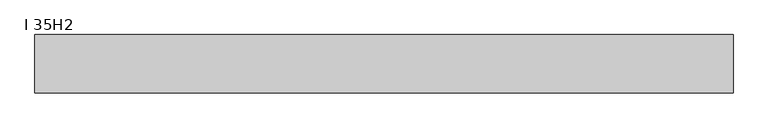
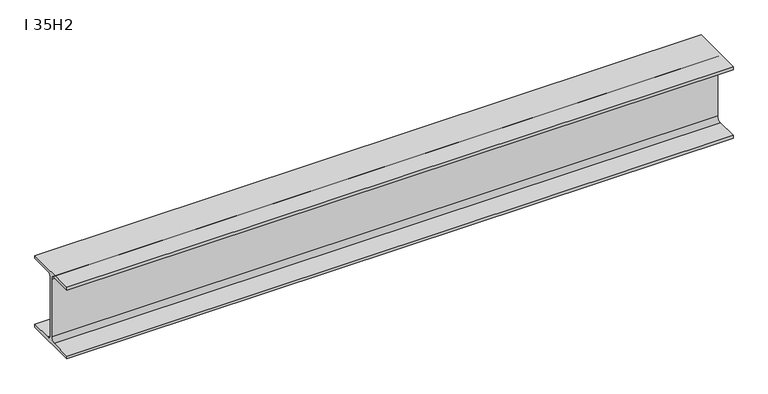
"""IFC4 building model written with IfcOpenShell, lengths in millimetres: beam geometry, Двутавр широкополочный (ГОСТ 26020-83) : I 35H2."""

import ifcopenshell
import ifcopenshell.guid

model = None  # the IFC model being written
_history = None  # IfcOwnerHistory: only IFC2X3 demands one
_inside = {}  # id of a spatial element -> (the spatial element, [elements in it])
_under = {}  # id of a project, library or spatial element -> (it, [spatial elements below it])
_declared = {}  # id of a project -> (the project, [libraries it declares])
_typed = {}  # id of a type object -> (the type object, [elements of that type])
_made_of = {}  # id of a material, layer set ... -> (it, [elements and type objects made of it])


def new_model(schema):
    """Start an empty IFC model of exactly this schema.

    Asked for "IFC4X3", IfcOpenShell would pick the latest addendum, in which some entities
    have other attributes; the version numbers below select the first issue.
    IFC2X3 requires an IfcOwnerHistory on every rooted entity: one is made here for all.
    """
    global model, _history
    if schema == "IFC4X3":
        model = ifcopenshell.file(schema_version=(4, 3, 0, 0))
    else:
        model = ifcopenshell.file(schema=schema)
    _inside.clear()
    _under.clear()
    _declared.clear()
    _typed.clear()
    _made_of.clear()
    _history = None
    if model.schema == "IFC2X3":
        org = make("IfcOrganization", Name="unknown")
        user = make(
            "IfcPersonAndOrganization",
            ThePerson=make("IfcPerson", FamilyName="unknown"),
            TheOrganization=org,
        )
        app = make(
            "IfcApplication",
            ApplicationDeveloper=org,
            Version="unknown",
            ApplicationFullName="unknown",
            ApplicationIdentifier="unknown",
        )
        _history = make(
            "IfcOwnerHistory",
            OwningUser=user,
            OwningApplication=app,
            ChangeAction="ADDED",
            CreationDate=0,
        )
    return model


def make(cls, **values):
    """One entity of the class cls with the attributes given. An attribute that is None is left unset."""
    return model.create_entity(
        cls, **{name: value for name, value in values.items() if value is not None}
    )


def rooted(cls, **values):
    """An entity with a GlobalId (a new one), such as an element, a storey or a relation."""
    return make(cls, GlobalId=ifcopenshell.guid.new(), OwnerHistory=_history, **values)


def si_unit(unit_type, name, prefix=None):
    """IfcSIUnit, for example si_unit("LENGTHUNIT", "METRE", prefix="MILLI")."""
    return make("IfcSIUnit", UnitType=unit_type, Prefix=prefix, Name=name)


def assignment(units):
    """IfcUnitAssignment: the units of a project."""
    return None if units is None else make("IfcUnitAssignment", Units=units)


def point(xyz):
    """IfcCartesianPoint."""
    return None if xyz is None else make("IfcCartesianPoint", Coordinates=xyz)


def direction(xyz):
    """IfcDirection."""
    return None if xyz is None else make("IfcDirection", DirectionRatios=xyz)


def frame(location, z_axis=None, x_axis=None):
    """IfcAxis2Placement3D, a coordinate frame: its origin and axes. An axis left out is left unset."""
    return make(
        "IfcAxis2Placement3D",
        Location=point(location),
        Axis=direction(z_axis),
        RefDirection=direction(x_axis),
    )


def frame_2d(location, x_axis=None):
    """IfcAxis2Placement2D, a coordinate frame in the plane: its origin and x axis."""
    return make(
        "IfcAxis2Placement2D", Location=point(location), RefDirection=direction(x_axis)
    )


def origin():
    """The frame at (0, 0, 0) with its axes left unset."""
    return frame((0.0, 0.0, 0.0))


def place(relative_to, where):
    """IfcLocalPlacement: puts the frame where relative to a parent placement (None: the world)."""
    return make(
        "IfcLocalPlacement", PlacementRelTo=relative_to, RelativePlacement=where
    )


def context(
    kind, dimensions, precision=None, world=None, true_north=None, identifier=None
):
    """IfcGeometricRepresentationContext, for example the 3D "Model" context."""
    return make(
        "IfcGeometricRepresentationContext",
        ContextIdentifier=identifier,
        ContextType=kind,
        CoordinateSpaceDimension=dimensions,
        Precision=precision,
        WorldCoordinateSystem=world,
        TrueNorth=true_north,
    )


def project(units=None, contexts=None):
    """IfcProject with its units and contexts."""
    return rooted(
        "IfcProject",
        Name="project",
        RepresentationContexts=contexts,
        UnitsInContext=assignment(units),
    )


def spatial(cls, under=None, at=None, **own):
    """A site, building, storey or space (cls), placed at a placement, below another one or the project."""
    s = rooted(cls, ObjectPlacement=at, **own)
    if under is not None:
        _under.setdefault(under.id(), (under, []))[1].append(s)
    return s


def polyline(points):
    """IfcPolyline through the points."""
    return make("IfcPolyline", Points=[point(p) for p in points])


def circle_curve(where, radius):
    """IfcCircle in the frame where."""
    return make("IfcCircle", Position=where, Radius=radius)


def trimmed(basis, trim1, trim2, sense, master):
    """IfcTrimmedCurve: the piece of a basis curve between two trims."""
    return make(
        "IfcTrimmedCurve",
        BasisCurve=basis,
        Trim1=trim1,
        Trim2=trim2,
        SenseAgreement=sense,
        MasterRepresentation=master,
    )


def segment(curve, same_sense, transition):
    """IfcCompositeCurveSegment."""
    return make(
        "IfcCompositeCurveSegment",
        Transition=transition,
        SameSense=same_sense,
        ParentCurve=curve,
    )


def composite_curve(segments, self_intersect=None):
    """IfcCompositeCurve: segments joined end to end."""
    return make("IfcCompositeCurve", Segments=segments, SelfIntersect=self_intersect)


def outline(outer, holes=None, kind="AREA"):
    """IfcArbitraryClosedProfileDef: a profile drawn as a closed curve; with holes, ...WithVoids."""
    if holes is None:
        return make("IfcArbitraryClosedProfileDef", ProfileType=kind, OuterCurve=outer)
    return make(
        "IfcArbitraryProfileDefWithVoids",
        ProfileType=kind,
        OuterCurve=outer,
        InnerCurves=holes,
    )


def extrude(swept, where, along, depth):
    """IfcExtrudedAreaSolid: the profile swept, set in the frame where, extruded along a direction by depth."""
    return make(
        "IfcExtrudedAreaSolid",
        SweptArea=swept,
        Position=where,
        ExtrudedDirection=direction(along),
        Depth=depth,
    )


def shape(context_of_items, identifier, shape_type, items):
    """IfcShapeRepresentation: the items that make up one representation, for example the "Body"."""
    return make(
        "IfcShapeRepresentation",
        ContextOfItems=context_of_items,
        RepresentationIdentifier=identifier,
        RepresentationType=shape_type,
        Items=items,
    )


def source(mapping_origin, context_of_items, identifier, shape_type, items):
    """IfcRepresentationMap: a shape defined once, which mapped items show again and again."""
    return make(
        "IfcRepresentationMap",
        MappingOrigin=mapping_origin,
        MappedRepresentation=shape(context_of_items, identifier, shape_type, items),
    )


def transform(
    local_origin,
    x_axis=None,
    y_axis=None,
    z_axis=None,
    scale=None,
    scale2=None,
    scale3=None,
    uniform=True,
):
    """IfcCartesianTransformationOperator3D, or its non-uniform kind. x_axis, y_axis, z_axis: its Axis1, 2, 3."""
    if uniform:
        return make(
            "IfcCartesianTransformationOperator3D",
            Axis1=direction(x_axis),
            Axis2=direction(y_axis),
            LocalOrigin=point(local_origin),
            Scale=scale,
            Axis3=direction(z_axis),
        )
    return make(
        "IfcCartesianTransformationOperator3DnonUniform",
        Axis1=direction(x_axis),
        Axis2=direction(y_axis),
        LocalOrigin=point(local_origin),
        Scale=scale,
        Axis3=direction(z_axis),
        Scale2=scale2,
        Scale3=scale3,
    )


def mapped(mapping_source, mapping_target):
    """IfcMappedItem: shows the shape of a source again, moved by a transform."""
    return make(
        "IfcMappedItem", MappingSource=mapping_source, MappingTarget=mapping_target
    )


def made_of(thing, what):
    """Note that an element or type object is made of a material, layer set ...; save() writes the relation."""
    if what is not None:
        _made_of.setdefault(what.id(), (what, []))[1].append(thing)
    return thing


def element(
    cls,
    number,
    at=None,
    inside=None,
    cuts=None,
    type_object=None,
    material=None,
    context=None,
    identifier="Body",
    shape_type=None,
    held_by="IfcProductDefinitionShape",
    body=None,
    shapes=None,
    **own,
):
    """One element of the class cls, such as IfcWall. Its Tag is "e" and its number.

    at: its placement. inside: the storey or other place that contains it. cuts: it is an
    opening in that element (IfcRelVoidsElement). A single representation is given by context,
    identifier, shape_type and body (its items); several are given by shapes. held_by: the class
    of the entity that holds the representations. save() writes the other relations.
    """
    e = rooted(cls, Tag="e%d" % number, ObjectPlacement=at, **own)
    if body is not None:
        shapes = [shape(context, identifier, shape_type, body)]
    if shapes is not None:
        e.Representation = make(held_by, Representations=shapes)
    if inside is not None:
        _inside.setdefault(inside.id(), (inside, []))[1].append(e)
    if cuts is not None:
        rooted(
            "IfcRelVoidsElement", RelatingBuildingElement=cuts, RelatedOpeningElement=e
        )
    if type_object is not None:
        _typed.setdefault(type_object.id(), (type_object, []))[1].append(e)
    return made_of(e, material)


def aggregate(whole, parts):
    """IfcRelAggregates: a whole, such as a stair, and the parts it consists of."""
    return rooted("IfcRelAggregates", RelatingObject=whole, RelatedObjects=parts)


def save(model, path):
    """Write the relations noted so far, then the file.

    IfcRelAggregates (storeys below a building ...), IfcRelContainedInSpatialStructure (elements
    in a storey), IfcRelDefinesByType, IfcRelAssociatesMaterial and IfcRelDeclares: one each for
    every whole, place, type object, material and project.
    """
    for whole, parts in _under.values():
        aggregate(whole, parts)
    for where, things in _inside.values():
        rooted(
            "IfcRelContainedInSpatialStructure",
            RelatedElements=things,
            RelatingStructure=where,
        )
    for kind, things in _typed.values():
        rooted("IfcRelDefinesByType", RelatedObjects=things, RelatingType=kind)
    for what, things in _made_of.values():
        rooted("IfcRelAssociatesMaterial", RelatedObjects=things, RelatingMaterial=what)
    for by, libraries in _declared.values():
        rooted("IfcRelDeclares", RelatingContext=by, RelatedDefinitions=libraries)
    model.write(path)


def i_35h2_abcca41d(model_context):
    return source(origin(), model_context, "Body", "SweptSolid", [
        extrude(outline(composite_curve([segment(polyline([(125.0, -156.5), (125.0, -170.5), (-125.0, -170.5), (-125.0, -156.5), (-25.0, -156.5)]), True, "CONTINUOUS"), segment(trimmed(circle_curve(frame_2d((-25.0, -136.5)), 20.0), [point((-25.0, -156.5))], [point((-5.0, -136.5))], True, "CARTESIAN"), True, "CONTINUOUS"), segment(polyline([(-5.0, -136.5), (-5.0, 136.5)]), True, "CONTINUOUS"), segment(trimmed(circle_curve(frame_2d((-25.0, 136.5)), 20.0), [point((-5.0, 136.5))], [point((-25.0, 156.5))], True, "CARTESIAN"), True, "CONTINUOUS"), segment(polyline([(-25.0, 156.5), (-125.0, 156.5), (-125.0, 170.5), (125.0, 170.5), (125.0, 156.5), (25.0, 156.5)]), True, "CONTINUOUS"), segment(trimmed(circle_curve(frame_2d((25.0, 136.5)), 20.0), [point((25.0, 156.5))], [point((5.0, 136.5))], True, "CARTESIAN"), True, "CONTINUOUS"), segment(polyline([(5.0, 136.5), (5.0, -136.5)]), True, "CONTINUOUS"), segment(trimmed(circle_curve(frame_2d((25.0, -136.5)), 20.0), [point((5.0, -136.5))], [point((25.0, -156.5))], True, "CARTESIAN"), True, "CONTINUOUS"), segment(polyline([(25.0, -156.5), (125.0, -156.5)]), True, "CONTINUOUS")], self_intersect=False)), frame((-1500.0, 0.0, 0.0), z_axis=(1.0, 0.0, 0.0), x_axis=(0.0, 1.0, 0.0)), (0.0, 0.0, 1.0), 3000.0),
    ])


if __name__ == "__main__":
    model = new_model("IFC4")
    model_context = context("Model", 3, world=origin())
    ifc_project = project(units=[si_unit("LENGTHUNIT", "METRE", prefix="MILLI")], contexts=[model_context])
    site = spatial("IfcSite", under=ifc_project)
    building = spatial("IfcBuilding", under=site)
    placement = place(None, origin())
    i_35h2_shape = i_35h2_abcca41d(model_context)
    element("IfcBeam", 1, ObjectType="Двутавр широкополочный (ГОСТ 26020-83) : I 35H2", at=placement, inside=building, context=model_context, shape_type="MappedRepresentation", body=[
        mapped(i_35h2_shape, transform((0.0, 0.0, 0.0), x_axis=(1.0, 0.0, 0.0), y_axis=(0.0, 1.0, 0.0), z_axis=(0.0, 0.0, 1.0))),
    ])
    save(model, "model.ifc")

# Revit data of these elements
# Type "Двутавр широкополочный (ГОСТ 26020-83) : I 35H2"
#   ra = 20 mm
#   W = 0.806107
#   Vz = 170.5 mm
#   Vy = 125 mm
#   Vpz = 170.5 mm
#   Vpy = 125 mm
#   Length [instance default] = 1500 mm
#   bf = 250 mm
#   d = 341 mm
#   tf = 14 mm
#   tw = 10 mm
#   A = 0.010474 m²
#   Structural Material [instance default] = Металл - Сталь - 345 МПa
#   Assembly Code = ""
# Element 1 (IfcBeam, "Двутавр широкополочный (ГОСТ 26020-83) : I 35H2")
#   Structural Material = C235
#   Materials on its faces: "C235"
# Materials
#   "Металл - Сталь - 345 МПa": class "Металл", colour RGB 247 247 247, transparency 0
#   "C235": class "Не назначено", colour RGB 0 0 0, transparency 0
